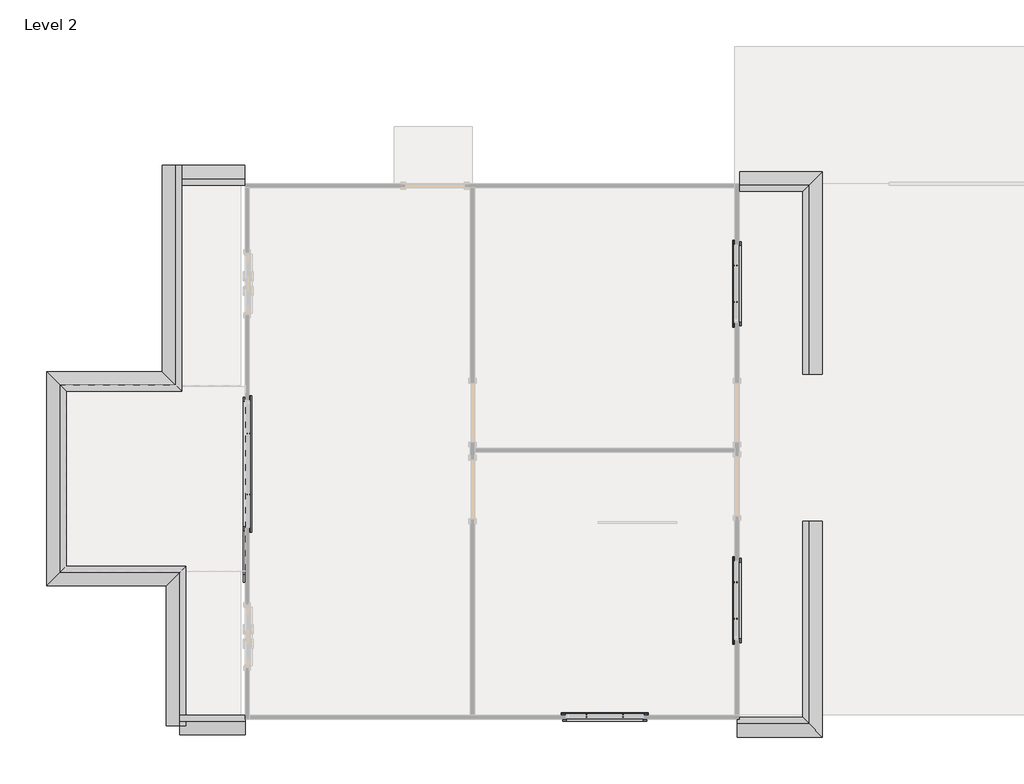
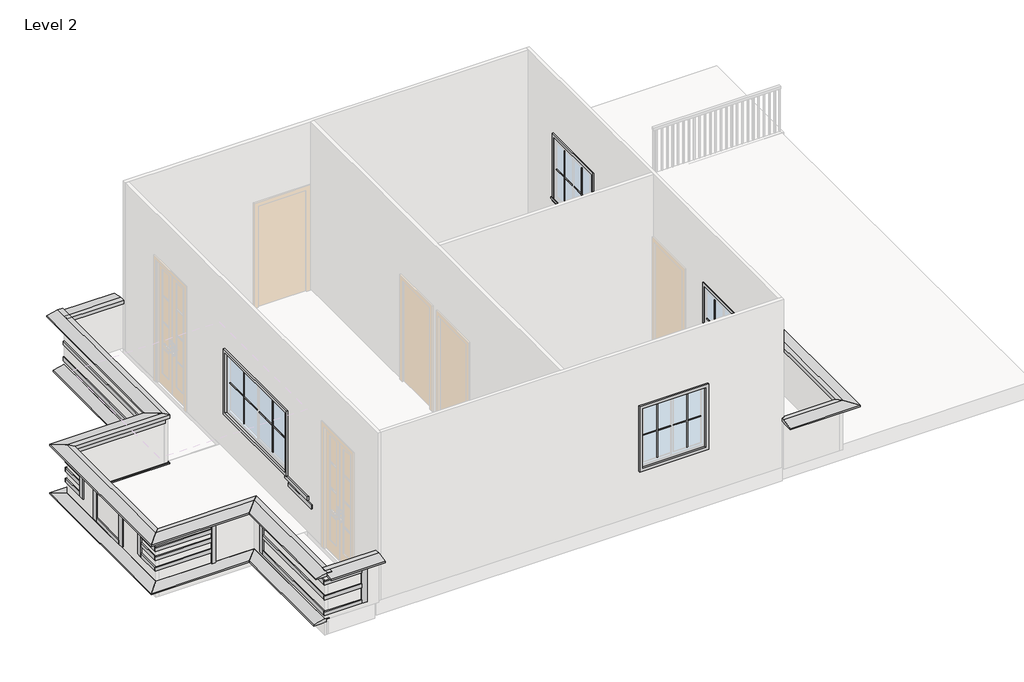
# One storey, part 2 of 2: 41 furniture elements, 34 proxies.
# Revit data of these elements (continued)
# Type "Muntin Pattern_2x2 : Muntin Pattern_2x2" (continued)
#   Width [instance default] = 4' - 0"
#   Thickness = 0' - 0 1/2"
#   Height [instance default] = 4' - 0"
#   Distance = 0' - 0 3/4"
#   Interior Material [instance default] = none
#   Exterior Material [instance default] = none
#   Default Elevation = 0
# Type "Trim-Window-Exterior-Flat : with Sill"
#   Trim Width = 0' - 2 1/4"
#   Trim Thickness_Picture Frame = 0' - 1 1/4"
#   Trim Thickness_with Sill = 0' - 0 3/4"
#   Sill Thickness = 0' - 1 1/4"
#   Opening Width [instance default] = 2' - 0"
#   Opening Height [instance default] = 3' - 0"
#   Default Elevation = 4' - 0"
#   Sill = yes
#   Picture Frame = no
#   Trim Material [instance default] = none
# Type "Trim-Window-Interior-Flat : Picture Frame"
#   Trim Thickness_Picture Frame = 0' - 1 1/4"
#   Trim Width = 0' - 2 1/4"
#   Trim Thickness_with Sill = 0' - 0 3/4"
#   Sill Thickness = 0' - 1 1/4"
#   Opening Width [instance default] = 2' - 0"
#   Opening Height [instance default] = 3' - 0"
#   Default Elevation = 4' - 0"
#   Sill = no
#   Picture Frame = yes
#   Trim Material [instance default] = none
# Type "M_Upper Cabinet-Filler-Wall : fhorizontal1"
#   Depth = 0' - 1"
#   Height = 0' - 3"
#   Top Of Cabinet = 6' - 6.74016"
#   Width = 1' - 6"
#   Cabinet Material = none
#   Default Elevation = 0
# Type "M_Upper Cabinet-Filler-Wall : Fverticle1"
#   Depth = 0' - 1"
#   Height = 1' - 6 7/16"
#   Top Of Cabinet = 6' - 6.74016"
#   Width = 0' - 4"
#   Cabinet Material = none
#   Default Elevation = 0
# Type "M_Upper Cabinet-Filler-Wall : fhorizontal2"
#   Depth = 0' - 1"
#   Height = 0' - 3"
#   Top Of Cabinet = 6' - 6.74016"
#   Width = 3' - 6"
#   Cabinet Material = none
#   Default Elevation = 0
# Type "M_Upper Cabinet-Filler-Wall : Fverticle1 3"
#   Depth = 0' - 1"
#   Height = 3' - 0"
#   Top Of Cabinet = 6' - 6.74016"
#   Width = 0' - 3"
#   Cabinet Material = none
#   Default Elevation = 0
# Type "M_Upper Cabinet-Filler-Wall : 75mm"
#   Depth = 0' - 1"
#   Height = 2' - 3"
#   Top Of Cabinet = 6' - 6.74016"
#   Width = 0' - 4"
#   Cabinet Material = none
#   Default Elevation = 0
# Type "M_Upper Cabinet-Filler-Wall : 75mm 2"
#   Depth = 0' - 3"
#   Height = 2' - 3"
#   Top Of Cabinet = 6' - 6 189/256"
#   Width = 0' - 4"
#   Cabinet Material = none
#   Default Elevation = 0
# Type "M_Upper Cabinet-Filler-Wall : horizontal"
#   Depth = 0' - 1"
#   Height = 0' - 3"
#   Top Of Cabinet = 6' - 6.74016"
#   Width = 2' - 4"
#   Cabinet Material = none
#   Default Elevation = 0
# Type "M_Upper Cabinet-Filler-Wall : horizontal 2"
#   Depth = 0' - 1"
#   Height = 0' - 3"
#   Top Of Cabinet = 6' - 6.74016"
#   Width = 2' - 5 1/2"
#   Cabinet Material = none
#   Default Elevation = 0
# Type "M_Upper Cabinet-Filler-Wall : horizontal 3"
#   Depth = 0' - 1"
#   Height = 0' - 3"
#   Top Of Cabinet = 6' - 6.74016"
#   Width = 6' - 6 1/2"
#   Cabinet Material = none
#   Default Elevation = 0
# Type "M_Upper Cabinet-Filler-Wall : horizontal 4"
#   Depth = 0' - 1"
#   Height = 0' - 3"
#   Top Of Cabinet = 6' - 6.74016"
#   Width = 9' - 5 1/2"
#   Cabinet Material = none
#   Default Elevation = 0
# Type "M_Upper Cabinet-Filler-Wall : horizontal 5"
#   Depth = 0' - 3"
#   Height = 0' - 3"
#   Top Of Cabinet = 6' - 6.74016"
#   Width = 2' - 5 1/2"
#   Cabinet Material = none
#   Default Elevation = 0
# Elements 1, 2, 3 (IfcBuildingElementProxy, "Cornice")
#   Phase Created = New Construction
#   Materials on its faces: "Phase - New"
# Elements 4, 6, 7, 10, 11 (IfcBuildingElementProxy, "Cornice")
#   Phase Created = New Construction
#   Materials on its faces: "Phase - New", "Vinyl Composition Tile"
# Elements 5, 8, 9 (IfcBuildingElementProxy, "Cornice")
#   Phase Created = New Construction
#   Materials on its faces: "Vinyl Composition Tile", "Phase - New"
# Elements 12, 13, 14, 15 (IfcBuildingElementProxy, "Cornice 3")
#   Phase Created = New Construction
#   Materials on its faces: "Phase - New", "Vinyl Composition Tile"
# Element 16 (IfcBuildingElementProxy, "Cornice 4")
#   Phase Created = New Construction
#   Materials on its faces: "Phase - New", "Vinyl Composition Tile"
# Elements 17, 18 (IfcBuildingElementProxy, "Cornice 4")
#   Phase Created = New Construction
#   Materials on its faces: "Phase - New"
# Elements 19, 20, 21, 22, 23, 24 (IfcBuildingElementProxy, "Muntin Pattern_2x2 : Muntin Pattern_2x2")
#   Width = 1' - 8 5/8"
#   Height = 3' - 6 1/4"
#   Interior Material = Wood - Stained
#   Exterior Material = Clad - White
#   Phase Created = New Construction
#   Materials on its faces: "Clad - White", "Wood - Stained"
# Elements 25, 26 (IfcBuildingElementProxy, "Muntin Pattern_2x2 : Muntin Pattern_2x2")
#   Width = 2' - 11 5/8"
#   Height = 3' - 6 1/4"
#   Interior Material = Wood - Stained
#   Exterior Material = Clad - White
#   Phase Created = New Construction
#   Materials on its faces: "Clad - White", "Wood - Stained"
# Elements 27, 28, 29 (IfcBuildingElementProxy, "Trim-Window-Exterior-Flat : with Sill")
#   Opening Width = 4' - 0"
#   Opening Height = 4' - 0"
#   Trim Material = Clad - White
#   Phase Created = New Construction
#   Materials on its faces: "Clad - White"
# Element 30 (IfcBuildingElementProxy, "Trim-Window-Exterior-Flat : with Sill")
#   Opening Width = 6' - 6"
#   Opening Height = 4' - 0"
#   Trim Material = Clad - White
#   Phase Created = New Construction
#   Materials on its faces: "Clad - White"
# Elements 31, 32, 33 (IfcBuildingElementProxy, "Trim-Window-Interior-Flat : Picture Frame")
#   Opening Width = 4' - 0"
#   Opening Height = 4' - 0"
#   Trim Material = Wood - Stained
#   Phase Created = New Construction
#   Materials on its faces: "Wood - Stained"
# Element 34 (IfcBuildingElementProxy, "Trim-Window-Interior-Flat : Picture Frame")
#   Opening Width = 6' - 6"
#   Opening Height = 4' - 0"
#   Trim Material = Wood - Stained
#   Phase Created = New Construction
#   Materials on its faces: "Wood - Stained"
# Elements 35, 36, 37, 38, 39, 40 (IfcFurniture, "M_Upper Cabinet-Filler-Wall : fhorizontal1")
#   Phase Created = New Construction
#   Materials on its faces: "Cabinets"
# Elements 41, 42 (IfcFurniture, "M_Upper Cabinet-Filler-Wall : Fverticle1")
#   Phase Created = New Construction
#   Materials on its faces: "Cabinets"
# Elements 43, 44, 45, 46, 47, 48 (IfcFurniture, "M_Upper Cabinet-Filler-Wall : fhorizontal2")
#   Phase Created = New Construction
#   Materials on its faces: "Cabinets"
# Elements 49, 50, 51, 52, 53 (IfcFurniture, "M_Upper Cabinet-Filler-Wall : Fverticle1 3")
#   Phase Created = New Construction
#   Materials on its faces: "Cabinets"
# Elements 54, 55, 56, 57 (IfcFurniture, "M_Upper Cabinet-Filler-Wall : 75mm")
#   Phase Created = New Construction
#   Materials on its faces: "Cabinets"
# Elements 58, 59 (IfcFurniture, "M_Upper Cabinet-Filler-Wall : 75mm 2")
#   Phase Created = New Construction
#   Materials on its faces: "Cabinets"
# Elements 60, 61, 62 (IfcFurniture, "M_Upper Cabinet-Filler-Wall : horizontal")
#   Phase Created = New Construction
#   Materials on its faces: "Cabinets"
# Elements 63, 64, 65, 66, 67 (IfcFurniture, "M_Upper Cabinet-Filler-Wall : horizontal 2")
#   Phase Created = New Construction
#   Materials on its faces: "Cabinets"
# Elements 68, 69, 70 (IfcFurniture, "M_Upper Cabinet-Filler-Wall : horizontal 3")
#   Phase Created = New Construction
#   Materials on its faces: "Cabinets"
# Elements 71, 72, 73 (IfcFurniture, "M_Upper Cabinet-Filler-Wall : horizontal 4")
#   Phase Created = New Construction
#   Materials on its faces: "Cabinets"
# Elements 74, 75 (IfcFurniture, "M_Upper Cabinet-Filler-Wall : horizontal 5")
#   Phase Created = New Construction
#   Materials on its faces: "Cabinets"
# Materials
#   "Phase - New": class "System", colour RGB 80 80 80, transparency 0, Cost = 0
#   "Vinyl Composition Tile": class "Generic", colour RGB 179 160 124, transparency 0, Description = "Vinyl Composition Tile", Cost = 0
#   "Clad - White": class "Wood", colour RGB 242 242 238, transparency 0, Cost = 0
#   "Wood - Stained": class "Wood", colour RGB 224 178 126, transparency 0, Cost = 0
#   "Cabinets": class "Miscellaneous", colour RGB 249 249 249, transparency 0
